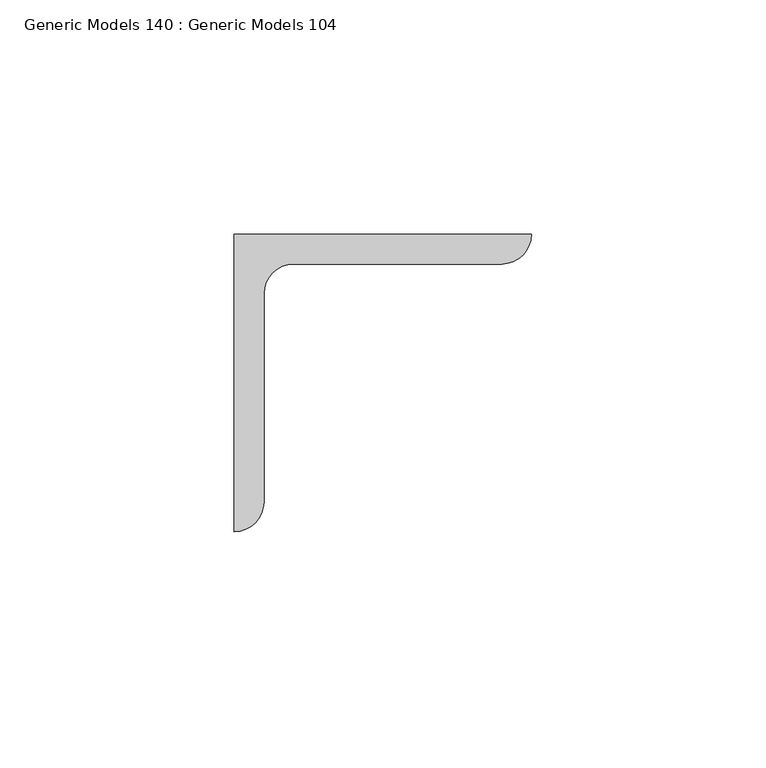
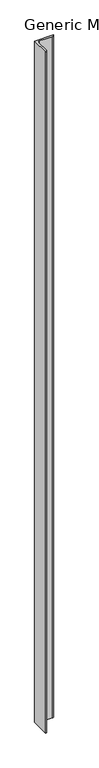
"""IFC4 building model written with IfcOpenShell, lengths in millimetres: proxy geometry, Generic Models 140 : Generic Models 104."""

from ifc_helpers import new_model, si_unit, point, frame, frame_2d, origin, place, context, project, spatial, polyline, circle_curve, trimmed, segment, composite_curve, outline, extrude, source, transform, mapped, element, save


def generic_models_140_generic_models_104_89fed35f(model_context):
    return source(origin(), model_context, "Body", "SweptSolid", [
        extrude(outline(composite_curve([segment(polyline([(31276.6040778, 41071.1196612), (31340.1040778, 41071.1196612)]), True, "CONTINUOUS"), segment(trimmed(circle_curve(frame_2d((31333.7540778, 41071.1196612)), 6.35), [point((31340.1040778, 41071.1196612))], [point((31333.7540778, 41064.7696612))], False, "CARTESIAN"), True, "CONTINUOUS"), segment(polyline([(31333.7540778, 41064.7696612), (31289.3040778, 41064.7696612)]), True, "CONTINUOUS"), segment(trimmed(circle_curve(frame_2d((31289.3040778, 41058.4196612)), 6.35), [point((31289.3040778, 41064.7696612))], [point((31282.9540778, 41058.4196612))], True, "CARTESIAN"), True, "CONTINUOUS"), segment(polyline([(31282.9540778, 41058.4196612), (31282.9540778, 41013.9696612)]), True, "CONTINUOUS"), segment(trimmed(circle_curve(frame_2d((31276.6040778, 41013.9696612)), 6.35), [point((31282.9540778, 41013.9696612))], [point((31276.6040778, 41007.6196612))], False, "CARTESIAN"), True, "CONTINUOUS"), segment(polyline([(31276.6040778, 41007.6196612), (31276.6040778, 41071.1196612)]), True, "CONTINUOUS")], self_intersect=False)), frame((0.0, 0.0, 266407.9), z_axis=(0.0, 0.0, 1.0), x_axis=(1.0, 0.0, 0.0)), (0.0, 0.0, 1.0), 2432.1044757),
    ])


if __name__ == "__main__":
    model = new_model("IFC4")
    model_context = context("Model", 3, world=origin())
    ifc_project = project(units=[si_unit("LENGTHUNIT", "METRE", prefix="MILLI")], contexts=[model_context])
    site = spatial("IfcSite", under=ifc_project)
    building = spatial("IfcBuilding", under=site)
    placement = place(None, origin())
    generic_models_140_generic_models_104_shape = generic_models_140_generic_models_104_89fed35f(model_context)
    element("IfcBuildingElementProxy", 1, Name="Generic Models 140 : Generic Models 104", ObjectType="Generic Models 140 : Generic Models 104", at=placement, inside=building, context=model_context, shape_type="MappedRepresentation", body=[
        mapped(generic_models_140_generic_models_104_shape, transform((0.0, 0.0, 0.0), x_axis=(1.0, 0.0, 0.0), y_axis=(0.0, 1.0, 0.0), z_axis=(0.0, 0.0, 1.0))),
    ])
    save(model, "model.ifc")

# Revit data of these elements
# Element 1 (IfcBuildingElementProxy, "Generic Models 140 : Generic Models 104")
#   Materials on its faces: "(2) BACK/BACK GALVANIZED ANGLES (2) L2 1/2 X 2 1/2 X 1/4\")"
# Materials
#   "(2) BACK/BACK GALVANIZED ANGLES (2) L2 1/2 X 2 1/2 X 1/4\")": class "Unassigned", colour RGB 211 211 211, transparency 0, Cost = 0
